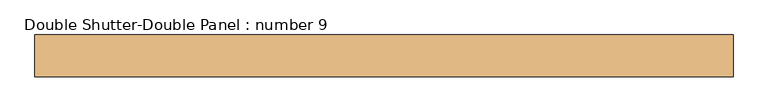
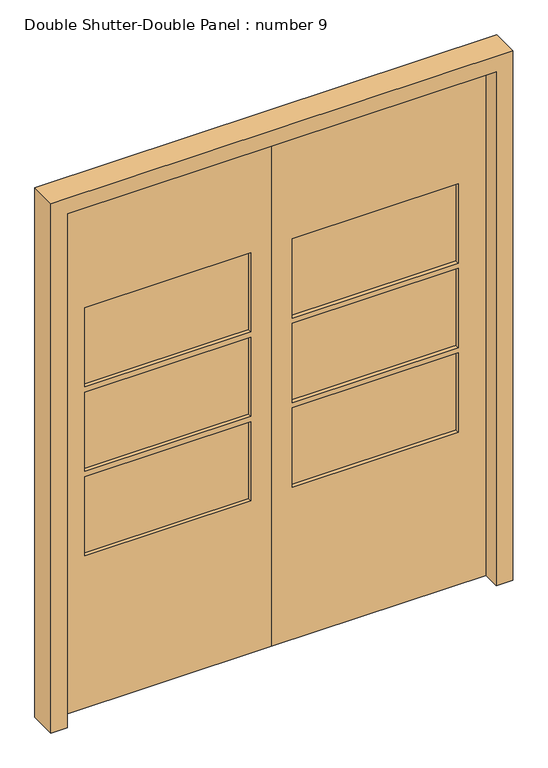
"""IFC4 building model written with IfcOpenShell, lengths in millimetres: door geometry, Double Shutter-Double Panel : number 9."""

from ifc_helpers import new_model, si_unit, frame, origin, place, context, project, spatial, polyline, outline, extrude, faceted_brep, source, transform, mapped, element, save


def double_shutter_double_panel_number_9_39cc3578(model_context):
    return source(origin(), model_context, "Body", "SolidModel", [
        extrude(outline(polyline([(678.2, 30.0), (75.0, 30.0), (75.0, 34.0), (678.2, 34.0), (678.2, 30.0)])), frame((0.0, 0.0, 250.0), z_axis=(0.0, 0.0, 1.0), x_axis=(1.0, 0.0, 0.0)), (0.0, 0.0, 1.0), 1622.0),
        extrude(outline(polyline([(-75.0, 30.0), (-678.2, 30.0), (-678.2, 34.0), (-75.0, 34.0), (-75.0, 30.0)])), frame((0.0, 0.0, 250.0), z_axis=(0.0, 0.0, 1.0), x_axis=(1.0, 0.0, 0.0)), (0.0, 0.0, 1.0), 1622.0),
        extrude(outline(polyline([(1987.0, 0.0), (1987.0, -793.2), (0.0, -793.2), (0.0, 0.0), (1987.0, 0.0)]), holes=[polyline([(1537.6, -678.2), (1537.6, -75.0), (1233.2, -75.0), (1233.2, -678.2), (1537.6, -678.2)]), polyline([(1213.2, -678.2), (1213.2, -75.0), (908.8, -75.0), (908.8, -678.2), (1213.2, -678.2)]), polyline([(888.8, -678.2), (888.8, -75.0), (584.4, -75.0), (584.4, -678.2), (888.8, -678.2)])]), frame((0.0, 15.0, 0.0), z_axis=(0.0, 1.0, 0.0), x_axis=(0.0, 0.0, 1.0)), (0.0, 0.0, 1.0), 35.0),
        extrude(outline(polyline([(1987.0, 0.0), (0.0, 0.0), (0.0, 793.2), (1987.0, 793.2), (1987.0, 0.0)]), holes=[polyline([(1537.6, 75.0), (1537.6, 678.2), (1233.2, 678.2), (1233.2, 75.0), (1537.6, 75.0)]), polyline([(1213.2, 75.0), (1213.2, 678.2), (908.8, 678.2), (908.8, 75.0), (1213.2, 75.0)]), polyline([(888.8, 75.0), (888.8, 678.2), (584.4, 678.2), (584.4, 75.0), (888.8, 75.0)])]), frame((0.0, 15.0, 0.0), z_axis=(0.0, 1.0, 0.0), x_axis=(0.0, 0.0, 1.0)), (0.0, 0.0, 1.0), 35.0),
        faceted_brep([(838.2, 50.0, 0.0), (838.2, -50.0, 0.0), (778.2, -50.0, 0.0), (778.2, 15.0, 0.0), (793.2, 15.0, 0.0), (793.2, 50.0, 0.0), (838.2, 50.0, 2032.0), (838.2, -50.0, 2032.0), (-838.2, -50.0, 2032.0), (-838.2, -50.0, 0.0), (-778.2, -50.0, 0.0), (-778.2, -50.0, 1972.0), (778.2, -50.0, 1972.0), (778.2, 15.0, 1972.0), (-778.2, 15.0, 1972.0), (-778.2, 15.0, 0.0), (-793.2, 15.0, 0.0), (-793.2, 15.0, 1987.0), (793.2, 15.0, 1987.0), (793.2, 50.0, 1987.0), (-793.2, 50.0, 1987.0), (-793.2, 50.0, 0.0), (-838.2, 50.0, 0.0), (-838.2, 50.0, 2032.0)], [[[0, 1, 2, 3, 4, 5]], [[1, 0, 6, 7]], [[2, 1, 7, 8, 9, 10, 11, 12]], [[3, 2, 12, 13]], [[4, 3, 13, 14, 15, 16, 17, 18]], [[5, 4, 18, 19]], [[0, 5, 19, 20, 21, 22, 23, 6]], [[7, 6, 23, 8]], [[13, 12, 11, 14]], [[19, 18, 17, 20]], [[22, 21, 16, 15, 10, 9]], [[8, 23, 22, 9]], [[14, 11, 10, 15]], [[20, 17, 16, 21]]]),
    ])


if __name__ == "__main__":
    model = new_model("IFC4")
    model_context = context("Model", 3, world=origin())
    ifc_project = project(units=[si_unit("LENGTHUNIT", "METRE", prefix="MILLI")], contexts=[model_context])
    site = spatial("IfcSite", under=ifc_project)
    building = spatial("IfcBuilding", under=site)
    placement = place(None, origin())
    double_shutter_double_panel_number_9_shape = double_shutter_double_panel_number_9_39cc3578(model_context)
    element("IfcDoor", 1, ObjectType="Double Shutter-Double Panel : number 9", at=placement, inside=building, context=model_context, shape_type="MappedRepresentation", body=[
        mapped(double_shutter_double_panel_number_9_shape, transform((0.0, 0.0, 0.0), x_axis=(1.0, 0.0, 0.0), y_axis=(0.0, 1.0, 0.0), z_axis=(0.0, 0.0, 1.0))),
    ])
    save(model, "model.ifc")

# Revit data of these elements
# Type "Double Shutter-Double Panel : number 9"
#   Type Mark = "90"
#   Analytic Construction = "<None>"
#   Top Rail = 0' - 3.93701"
#   Stile = 0' - 3.93701"
#   Frame Width = 0' - 2.3622"
#   Height = 6' - 8"
#   Width = 5' - 6"
#   Frame Depth = 0' - 3.93701"
#   Bottom Rail = 0' - 9.84252"
#   Define Thermal Properties by = 1
#   Material of Glass panel = Glass - Frosted
#   Material of Frame/Shutter = Frame /Shutter
#   Function = (empty or 0)
#   Wall Closure = (empty or 0)
#   Assembly Code = ""
# Element 1 (IfcDoor, "Double Shutter-Double Panel : number 9")
#   Materials on its faces: "Frame /Shutter", "Glass - Frosted"
# Materials
#   "Glass - Frosted": class "Glass", colour RGB 250 244 225, transparency 0.51
#   "Frame /Shutter": class "Wood", colour RGB 145 112 90, transparency 0
